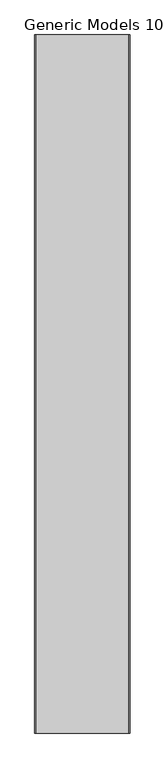
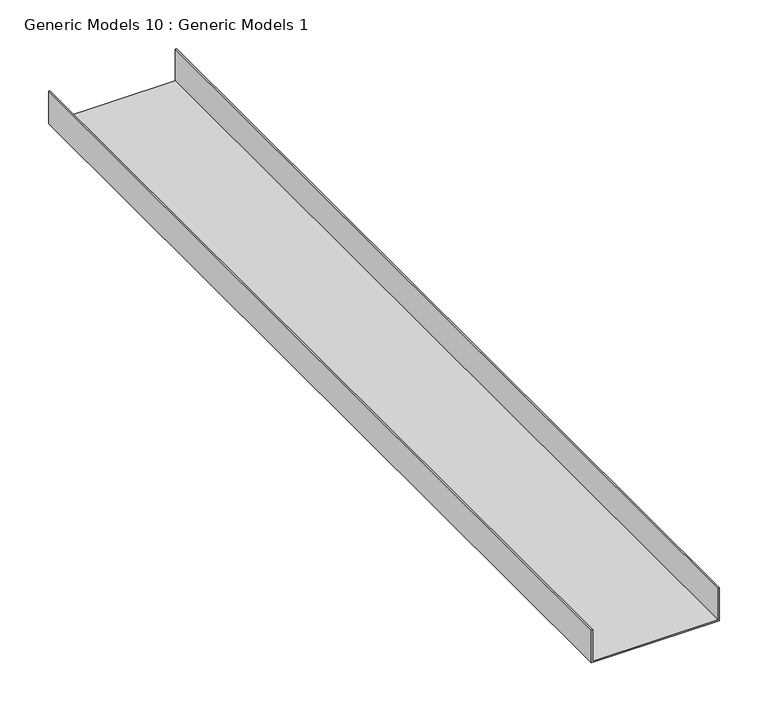
"""IFC4 building model written with IfcOpenShell, lengths in millimetres: proxy geometry, Generic Models 10 : Generic Models 1."""

from ifc_helpers import new_model, si_unit, frame, origin, place, context, project, spatial, polyline, outline, extrude, source, transform, mapped, element, save


def generic_models_10_generic_models_1_b874e651(model_context):
    return source(origin(), model_context, "Body", "SweptSolid", [
        extrude(outline(polyline([(2495.55, 55668.3562571), (2495.55, 55820.7562571), (2536.825, 55820.7562571), (2536.825, 55819.1687571), (2497.1375, 55819.1687571), (2497.1375, 55669.9437571), (2536.825, 55669.9437571), (2536.825, 55668.3562571), (2495.55, 55668.3562571)])), frame((0.0, 36117.4598594, 0.0), z_axis=(0.0, 1.0, 0.0), x_axis=(0.0, 0.0, 1.0)), (0.0, 0.0, 1.0), 1117.6),
    ])


if __name__ == "__main__":
    model = new_model("IFC4")
    model_context = context("Model", 3, world=origin())
    ifc_project = project(units=[si_unit("LENGTHUNIT", "METRE", prefix="MILLI")], contexts=[model_context])
    site = spatial("IfcSite", under=ifc_project)
    building = spatial("IfcBuilding", under=site)
    placement = place(None, origin())
    generic_models_10_generic_models_1_shape = generic_models_10_generic_models_1_b874e651(model_context)
    element("IfcBuildingElementProxy", 1, Name="Generic Models 10 : Generic Models 1", ObjectType="Generic Models 10 : Generic Models 1", at=placement, inside=building, context=model_context, shape_type="MappedRepresentation", body=[
        mapped(generic_models_10_generic_models_1_shape, transform((0.0, 0.0, 0.0), x_axis=(1.0, 0.0, 0.0), y_axis=(0.0, 1.0, 0.0), z_axis=(0.0, 0.0, 1.0))),
    ])
    save(model, "model.ifc")

# Revit data of these elements
# Element 1 (IfcBuildingElementProxy, "Generic Models 10 : Generic Models 1")
#   Materials on its faces: "METAL STUDS"
# Materials
#   "METAL STUDS": class "Unassigned", colour RGB 210 209 208, transparency 0, Keynote = "M05121300.02", Cost = 0
